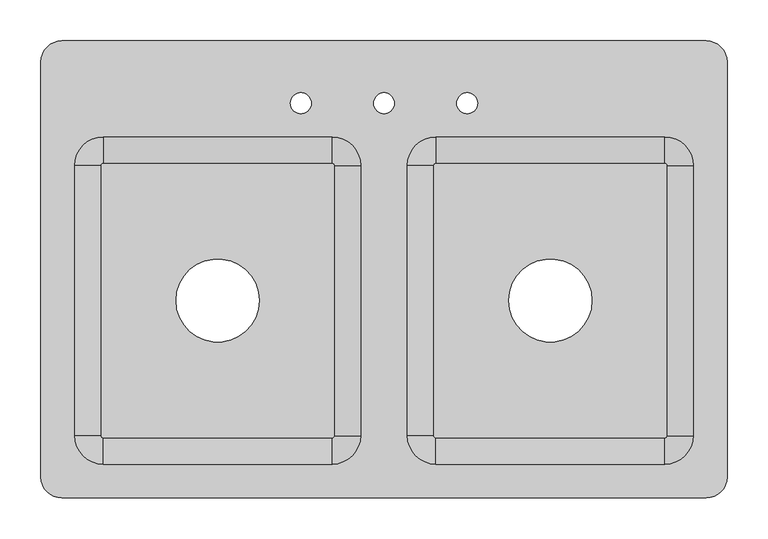
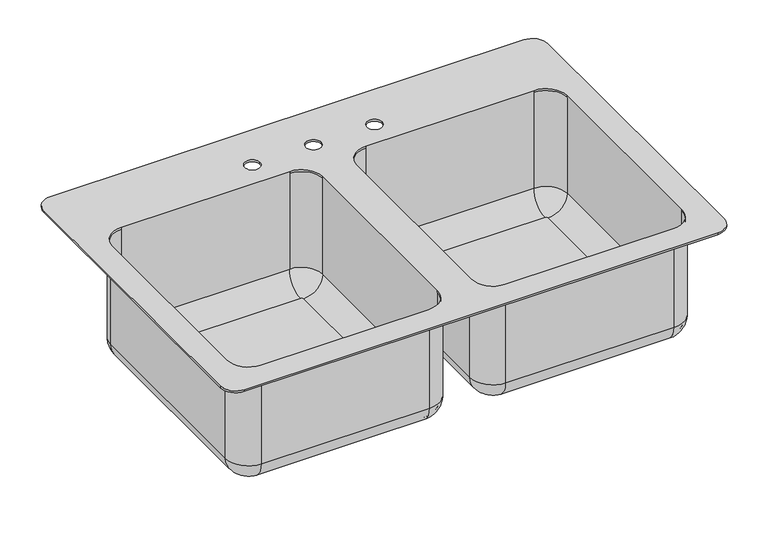
"""IFC4 building model written with IfcOpenShell, lengths in millimetres: proxy geometry, Double_Bowl_Kitchen_Sink_w_Delta_Faucet_and_drains_14175 : Double_Bowl_Kitchen_Sink_w_Delta_Faucet_and_drains_14175."""

import ifcopenshell
import ifcopenshell.guid

model = None  # the IFC model being written
_history = None  # IfcOwnerHistory: only IFC2X3 demands one
_inside = {}  # id of a spatial element -> (the spatial element, [elements in it])
_under = {}  # id of a project, library or spatial element -> (it, [spatial elements below it])
_declared = {}  # id of a project -> (the project, [libraries it declares])
_typed = {}  # id of a type object -> (the type object, [elements of that type])
_made_of = {}  # id of a material, layer set ... -> (it, [elements and type objects made of it])


def new_model(schema):
    """Start an empty IFC model of exactly this schema.

    Asked for "IFC4X3", IfcOpenShell would pick the latest addendum, in which some entities
    have other attributes; the version numbers below select the first issue.
    IFC2X3 requires an IfcOwnerHistory on every rooted entity: one is made here for all.
    """
    global model, _history
    if schema == "IFC4X3":
        model = ifcopenshell.file(schema_version=(4, 3, 0, 0))
    else:
        model = ifcopenshell.file(schema=schema)
    _inside.clear()
    _under.clear()
    _declared.clear()
    _typed.clear()
    _made_of.clear()
    _history = None
    if model.schema == "IFC2X3":
        org = make("IfcOrganization", Name="unknown")
        user = make(
            "IfcPersonAndOrganization",
            ThePerson=make("IfcPerson", FamilyName="unknown"),
            TheOrganization=org,
        )
        app = make(
            "IfcApplication",
            ApplicationDeveloper=org,
            Version="unknown",
            ApplicationFullName="unknown",
            ApplicationIdentifier="unknown",
        )
        _history = make(
            "IfcOwnerHistory",
            OwningUser=user,
            OwningApplication=app,
            ChangeAction="ADDED",
            CreationDate=0,
        )
    return model


def make(cls, **values):
    """One entity of the class cls with the attributes given. An attribute that is None is left unset."""
    return model.create_entity(
        cls, **{name: value for name, value in values.items() if value is not None}
    )


def rooted(cls, **values):
    """An entity with a GlobalId (a new one), such as an element, a storey or a relation."""
    return make(cls, GlobalId=ifcopenshell.guid.new(), OwnerHistory=_history, **values)


def si_unit(unit_type, name, prefix=None):
    """IfcSIUnit, for example si_unit("LENGTHUNIT", "METRE", prefix="MILLI")."""
    return make("IfcSIUnit", UnitType=unit_type, Prefix=prefix, Name=name)


def assignment(units):
    """IfcUnitAssignment: the units of a project."""
    return None if units is None else make("IfcUnitAssignment", Units=units)


def point(xyz):
    """IfcCartesianPoint."""
    return None if xyz is None else make("IfcCartesianPoint", Coordinates=xyz)


def direction(xyz):
    """IfcDirection."""
    return None if xyz is None else make("IfcDirection", DirectionRatios=xyz)


def frame(location, z_axis=None, x_axis=None):
    """IfcAxis2Placement3D, a coordinate frame: its origin and axes. An axis left out is left unset."""
    return make(
        "IfcAxis2Placement3D",
        Location=point(location),
        Axis=direction(z_axis),
        RefDirection=direction(x_axis),
    )


def origin():
    """The frame at (0, 0, 0) with its axes left unset."""
    return frame((0.0, 0.0, 0.0))


def place(relative_to, where):
    """IfcLocalPlacement: puts the frame where relative to a parent placement (None: the world)."""
    return make(
        "IfcLocalPlacement", PlacementRelTo=relative_to, RelativePlacement=where
    )


def context(
    kind, dimensions, precision=None, world=None, true_north=None, identifier=None
):
    """IfcGeometricRepresentationContext, for example the 3D "Model" context."""
    return make(
        "IfcGeometricRepresentationContext",
        ContextIdentifier=identifier,
        ContextType=kind,
        CoordinateSpaceDimension=dimensions,
        Precision=precision,
        WorldCoordinateSystem=world,
        TrueNorth=true_north,
    )


def project(units=None, contexts=None):
    """IfcProject with its units and contexts."""
    return rooted(
        "IfcProject",
        Name="project",
        RepresentationContexts=contexts,
        UnitsInContext=assignment(units),
    )


def spatial(cls, under=None, at=None, **own):
    """A site, building, storey or space (cls), placed at a placement, below another one or the project."""
    s = rooted(cls, ObjectPlacement=at, **own)
    if under is not None:
        _under.setdefault(under.id(), (under, []))[1].append(s)
    return s


def polyline(points):
    """IfcPolyline through the points."""
    return make("IfcPolyline", Points=[point(p) for p in points])


def circle_curve(where, radius):
    """IfcCircle in the frame where."""
    return make("IfcCircle", Position=where, Radius=radius)


def ellipse_curve(where, semi_axis1, semi_axis2):
    """IfcEllipse in the frame where."""
    return make(
        "IfcEllipse", Position=where, SemiAxis1=semi_axis1, SemiAxis2=semi_axis2
    )


def trimmed(basis, trim1, trim2, sense, master):
    """IfcTrimmedCurve: the piece of a basis curve between two trims."""
    return make(
        "IfcTrimmedCurve",
        BasisCurve=basis,
        Trim1=trim1,
        Trim2=trim2,
        SenseAgreement=sense,
        MasterRepresentation=master,
    )


def shape(context_of_items, identifier, shape_type, items):
    """IfcShapeRepresentation: the items that make up one representation, for example the "Body"."""
    return make(
        "IfcShapeRepresentation",
        ContextOfItems=context_of_items,
        RepresentationIdentifier=identifier,
        RepresentationType=shape_type,
        Items=items,
    )


def source(mapping_origin, context_of_items, identifier, shape_type, items):
    """IfcRepresentationMap: a shape defined once, which mapped items show again and again."""
    return make(
        "IfcRepresentationMap",
        MappingOrigin=mapping_origin,
        MappedRepresentation=shape(context_of_items, identifier, shape_type, items),
    )


def transform(
    local_origin,
    x_axis=None,
    y_axis=None,
    z_axis=None,
    scale=None,
    scale2=None,
    scale3=None,
    uniform=True,
):
    """IfcCartesianTransformationOperator3D, or its non-uniform kind. x_axis, y_axis, z_axis: its Axis1, 2, 3."""
    if uniform:
        return make(
            "IfcCartesianTransformationOperator3D",
            Axis1=direction(x_axis),
            Axis2=direction(y_axis),
            LocalOrigin=point(local_origin),
            Scale=scale,
            Axis3=direction(z_axis),
        )
    return make(
        "IfcCartesianTransformationOperator3DnonUniform",
        Axis1=direction(x_axis),
        Axis2=direction(y_axis),
        LocalOrigin=point(local_origin),
        Scale=scale,
        Axis3=direction(z_axis),
        Scale2=scale2,
        Scale3=scale3,
    )


def mapped(mapping_source, mapping_target):
    """IfcMappedItem: shows the shape of a source again, moved by a transform."""
    return make(
        "IfcMappedItem", MappingSource=mapping_source, MappingTarget=mapping_target
    )


def made_of(thing, what):
    """Note that an element or type object is made of a material, layer set ...; save() writes the relation."""
    if what is not None:
        _made_of.setdefault(what.id(), (what, []))[1].append(thing)
    return thing


def element(
    cls,
    number,
    at=None,
    inside=None,
    cuts=None,
    type_object=None,
    material=None,
    context=None,
    identifier="Body",
    shape_type=None,
    held_by="IfcProductDefinitionShape",
    body=None,
    shapes=None,
    **own,
):
    """One element of the class cls, such as IfcWall. Its Tag is "e" and its number.

    at: its placement. inside: the storey or other place that contains it. cuts: it is an
    opening in that element (IfcRelVoidsElement). A single representation is given by context,
    identifier, shape_type and body (its items); several are given by shapes. held_by: the class
    of the entity that holds the representations. save() writes the other relations.
    """
    e = rooted(cls, Tag="e%d" % number, ObjectPlacement=at, **own)
    if body is not None:
        shapes = [shape(context, identifier, shape_type, body)]
    if shapes is not None:
        e.Representation = make(held_by, Representations=shapes)
    if inside is not None:
        _inside.setdefault(inside.id(), (inside, []))[1].append(e)
    if cuts is not None:
        rooted(
            "IfcRelVoidsElement", RelatingBuildingElement=cuts, RelatedOpeningElement=e
        )
    if type_object is not None:
        _typed.setdefault(type_object.id(), (type_object, []))[1].append(e)
    return made_of(e, material)


def aggregate(whole, parts):
    """IfcRelAggregates: a whole, such as a stair, and the parts it consists of."""
    return rooted("IfcRelAggregates", RelatingObject=whole, RelatedObjects=parts)


def save(model, path):
    """Write the relations noted so far, then the file.

    IfcRelAggregates (storeys below a building ...), IfcRelContainedInSpatialStructure (elements
    in a storey), IfcRelDefinesByType, IfcRelAssociatesMaterial and IfcRelDeclares: one each for
    every whole, place, type object, material and project.
    """
    for whole, parts in _under.values():
        aggregate(whole, parts)
    for where, things in _inside.values():
        rooted(
            "IfcRelContainedInSpatialStructure",
            RelatedElements=things,
            RelatingStructure=where,
        )
    for kind, things in _typed.values():
        rooted("IfcRelDefinesByType", RelatedObjects=things, RelatingType=kind)
    for what, things in _made_of.values():
        rooted("IfcRelAssociatesMaterial", RelatedObjects=things, RelatingMaterial=what)
    for by, libraries in _declared.values():
        rooted("IfcRelDeclares", RelatingContext=by, RelatedDefinitions=libraries)
    model.write(path)


def plane_surface(at):
    """IfcPlane: the flat surface through the origin of the frame at, square to its z axis."""
    return make("IfcPlane", Position=at)


def cylinder_surface(at, radius):
    """IfcCylindricalSurface: all points at the distance radius from the z axis of the frame at."""
    return make("IfcCylindricalSurface", Position=at, Radius=radius)


def revolved_surface(curve, axis_point, axis_direction):
    """IfcSurfaceOfRevolution: the curve turned about the line through axis_point along axis_direction."""
    return make(
        "IfcSurfaceOfRevolution",
        SweptCurve=make("IfcArbitraryOpenProfileDef", ProfileType="CURVE", Curve=curve),
        AxisPosition=make("IfcAxis1Placement", Location=point(axis_point), Axis=direction(axis_direction)),
    )


def advanced_brep(points, edges, surfaces, faces):
    """IfcAdvancedBrep: a solid bounded by faces that lie on surfaces and meet in shared edges.

    An edge is (start, end): straight between two places in points (the first is 0);
    or (start, end, curve); or (start, end, curve, False) where it runs against its curve.
    A face is (place in surfaces, loops), or (place, loops, False) where it looks against
    its surface's normal. A loop lists edges by number (the first is 1), with a minus sign
    where the edge is run from its end to its start. The first loop is the outer one.
    """
    corners = [point(p) for p in points]
    vertices = [make("IfcVertexPoint", VertexGeometry=c) for c in corners]
    made = []
    for start, end, *more in edges:
        made.append(
            make(
                "IfcEdgeCurve",
                EdgeStart=vertices[start],
                EdgeEnd=vertices[end],
                EdgeGeometry=more[0] if more else make("IfcPolyline", Points=[corners[start], corners[end]]),
                SameSense=more[1] if len(more) > 1 else True,
            )
        )
    hull = []
    for where, loops, *sense in faces:
        bounds = []
        for j, loop in enumerate(loops):
            ring = [make("IfcOrientedEdge", EdgeElement=made[abs(k) - 1], Orientation=k > 0) for k in loop]
            bounds.append(
                make(
                    "IfcFaceOuterBound" if j == 0 else "IfcFaceBound",
                    Bound=make("IfcEdgeLoop", EdgeList=ring),
                    Orientation=True,
                )
            )
        hull.append(make("IfcAdvancedFace", Bounds=bounds, FaceSurface=surfaces[where], SameSense=sense[0] if sense else True))
    return make("IfcAdvancedBrep", Outer=make("IfcClosedShell", CfsFaces=hull))


def specialty_equipment_74882aa0(model_context):
    return source(origin(), model_context, "Body", "AdvancedBrep", [
        advanced_brep(
        [(342.9, 161.925, 0.0), (342.9, 161.925, -168.275), (377.825, 127.0, -168.275), (377.825, 127.0, 0.0), (381.0, 127.0, -168.275), (342.9, 165.1, -168.275), (342.9, 165.1, 0.0), (381.0, 127.0, 0.0), (346.075, 127.0, -203.2), (342.9, 130.175, -203.2), (342.9, 130.175, -200.025), (346.075, 127.0, -200.025), (381.0, -203.2, 0.0), (381.0, -203.2, -168.275), (346.075, -203.2, -203.2), (346.075, -203.2, -200.025), (377.825, -203.2, -168.275), (377.825, -203.2, 0.0), (342.9, -238.125, -168.275), (342.9, -238.125, 0.0), (342.9, -241.3, 0.0), (342.9, -241.3, -168.275), (342.9, -206.375, -203.2), (342.9, -206.375, -200.025), (63.5, -241.3, 0.0), (63.5, -241.3, -168.275), (63.5, -206.375, -203.2), (63.5, -206.375, -200.025), (63.5, -238.125, -168.275), (63.5, -238.125, 0.0), (28.575, -203.2, -168.275), (28.575, -203.2, 0.0), (25.4, -203.2, 0.0), (25.4, -203.2, -168.275), (60.325, -203.2, -203.2), (60.325, -203.2, -200.025), (25.4, 127.0, 0.0), (25.4, 127.0, -168.275), (60.325, 127.0, -203.2), (60.325, 127.0, -200.025), (28.575, 127.0, -168.275), (28.575, 127.0, 0.0), (63.5, 161.925, -168.275), (63.5, 161.925, 0.0), (63.5, 165.1, 0.0), (63.5, 165.1, -168.275), (63.5, 130.175, -203.2), (63.5, 130.175, -200.025), (393.7, 279.4, 3.175), (-393.7, 279.4, 3.175), (-419.1, 254.0, 3.175), (-419.1, -254.0, 3.175), (-393.7, -279.4, 3.175), (393.7, -279.4, 3.175), (419.1, -254.0, 3.175), (419.1, 254.0, 3.175), (-88.9, 203.2, 3.175), (-114.3, 203.2, 3.175), (12.7, 203.2, 3.175), (-12.7, 203.2, 3.175), (114.3, 203.2, 3.175), (88.9, 203.2, 3.175), (-342.9, 161.925, 3.175), (-63.5, 161.925, 3.175), (-28.575, 127.0, 3.175), (-28.575, -203.2, 3.175), (-63.5, -238.125, 3.175), (-342.9, -238.125, 3.175), (-377.825, -203.2, 3.175), (-377.825, 127.0, 3.175), (28.575, 127.0, 3.175), (63.5, 161.925, 3.175), (342.9, 161.925, 3.175), (377.825, 127.0, 3.175), (377.825, -203.2, 3.175), (342.9, -238.125, 3.175), (63.5, -238.125, 3.175), (28.575, -203.2, 3.175), (393.7, 279.4, 0.0), (419.1, 254.0, 0.0), (419.1, -254.0, 0.0), (393.7, -279.4, 0.0), (-393.7, -279.4, 0.0), (-419.1, -254.0, 0.0), (-419.1, 254.0, 0.0), (-393.7, 279.4, 0.0), (-114.3, 203.2, 0.0), (-88.9, 203.2, 0.0), (-12.7, 203.2, 0.0), (12.7, 203.2, 0.0), (88.9, 203.2, 0.0), (114.3, 203.2, 0.0), (-25.4, 127.0, 0.0), (-63.5, 165.1, 0.0), (-342.9, 165.1, 0.0), (-381.0, 127.0, 0.0), (-381.0, -203.2, 0.0), (-342.9, -241.3, 0.0), (-63.5, -241.3, 0.0), (-25.4, -203.2, 0.0), (-63.5, 161.925, 0.0), (-342.9, 161.925, 0.0), (-342.9, 161.925, -168.275), (-63.5, 161.925, -168.275), (-377.825, 127.0, 0.0), (-377.825, -203.2, 0.0), (-377.825, -203.2, -168.275), (-377.825, 127.0, -168.275), (-342.9, -238.125, 0.0), (-63.5, -238.125, 0.0), (-63.5, -238.125, -168.275), (-342.9, -238.125, -168.275), (-28.575, -203.2, 0.0), (-28.575, 127.0, 0.0), (-28.575, 127.0, -168.275), (-28.575, -203.2, -168.275), (-25.4, 127.0, -168.275), (-63.5, 165.1, -168.275), (-60.325, 127.0, -203.2), (-63.5, 130.175, -203.2), (-63.5, 130.175, -200.025), (-60.325, 127.0, -200.025), (-25.4, -203.2, -168.275), (-60.325, -203.2, -203.2), (-60.325, -203.2, -200.025), (-63.5, -241.3, -168.275), (-63.5, -206.375, -203.2), (-63.5, -206.375, -200.025), (-342.9, -241.3, -168.275), (-342.9, -206.375, -203.2), (-342.9, -206.375, -200.025), (-381.0, -203.2, -168.275), (-346.075, -203.2, -203.2), (-346.075, -203.2, -200.025), (-381.0, 127.0, -168.275), (-346.075, 127.0, -203.2), (-346.075, 127.0, -200.025), (-342.9, 165.1, -168.275), (-342.9, 130.175, -203.2), (-342.9, 130.175, -200.025), (152.4, -38.1, -200.025), (254.0, -38.1, -200.025), (-254.0, -38.1, -200.025), (-152.4, -38.1, -200.025), (254.0, -38.1, -203.2), (152.4, -38.1, -203.2), (-152.4, -38.1, -203.2), (-254.0, -38.1, -203.2)],
        [
            (0, 1),
            (1, 2, circle_curve(frame((342.9, 127.0, -168.275), z_axis=(0.0, 0.0, -1.0), x_axis=(0.0, 1.0, 0.0)), 34.925)),
            (2, 3),
            (3, 0, circle_curve(frame((342.9, 127.0, 0.0), z_axis=(0.0, 0.0, 1.0), x_axis=(0.0, 1.0, 0.0)), 34.925)),
            (4, 5, circle_curve(frame((342.9, 127.0, -168.275), z_axis=(0.0, 0.0, 1.0), x_axis=(0.0, 1.0, 0.0)), 38.1)),
            (5, 6),
            (6, 7, circle_curve(frame((342.9, 127.0, 0.0), z_axis=(0.0, 0.0, -1.0), x_axis=(0.0, 1.0, 0.0)), 38.1)),
            (7, 4),
            (4, 8, circle_curve(frame((346.075, 127.0, -168.275), z_axis=(0.0, 1.0, 0.0), x_axis=(1.0, 0.0, 0.0)), 34.925)),
            (8, 9, circle_curve(frame((342.9, 127.0, -203.2), z_axis=(0.0, 0.0, 1.0), x_axis=(0.0, 1.0, 0.0)), 3.175)),
            (9, 5, circle_curve(frame((342.9, 130.175, -168.275), z_axis=(1.0, 0.0, 0.0), x_axis=(0.0, 1.0, 0.0)), 34.925)),
            (1, 10, circle_curve(frame((342.9, 130.175, -168.275), z_axis=(-1.0, 0.0, 0.0), x_axis=(0.0, 1.0, 0.0)), 31.75)),
            (10, 11, circle_curve(frame((342.9, 127.0, -200.025), z_axis=(0.0, 0.0, -1.0), x_axis=(0.0, 1.0, 0.0)), 3.175)),
            (11, 2, circle_curve(frame((346.075, 127.0, -168.275), z_axis=(0.0, -1.0, 0.0), x_axis=(1.0, 0.0, 0.0)), 31.75)),
            (7, 12),
            (12, 13),
            (13, 4),
            (13, 14, circle_curve(frame((346.075, -203.2, -168.275), z_axis=(0.0, 1.0, 0.0), x_axis=(1.0, 0.0, 0.0)), 34.925)),
            (14, 8),
            (11, 15),
            (15, 16, circle_curve(frame((346.075, -203.2, -168.275), z_axis=(0.0, -1.0, 0.0), x_axis=(1.0, 0.0, 0.0)), 31.75)),
            (16, 2),
            (17, 16),
            (16, 18, circle_curve(frame((342.9, -203.2, -168.275), z_axis=(0.0, 0.0, -1.0), x_axis=(1.0, 0.0, 0.0)), 34.925)),
            (18, 19),
            (19, 17, circle_curve(frame((342.9, -203.2, 0.0), z_axis=(0.0, 0.0, 1.0), x_axis=(1.0, 0.0, 0.0)), 34.925)),
            (12, 20, circle_curve(frame((342.9, -203.2, 0.0), z_axis=(0.0, 0.0, -1.0), x_axis=(1.0, 0.0, 0.0)), 38.1)),
            (20, 21),
            (21, 13, circle_curve(frame((342.9, -203.2, -168.275), z_axis=(0.0, 0.0, 1.0), x_axis=(1.0, 0.0, 0.0)), 38.1)),
            (21, 22, circle_curve(frame((342.9, -206.375, -168.275), z_axis=(1.0, 0.0, 0.0), x_axis=(0.0, -1.0, 0.0)), 34.925)),
            (22, 14, circle_curve(frame((342.9, -203.2, -203.2), z_axis=(0.0, 0.0, 1.0), x_axis=(1.0, 0.0, 0.0)), 3.175)),
            (15, 23, circle_curve(frame((342.9, -203.2, -200.025), z_axis=(0.0, 0.0, -1.0), x_axis=(1.0, 0.0, 0.0)), 3.175)),
            (23, 18, circle_curve(frame((342.9, -206.375, -168.275), z_axis=(-1.0, 0.0, 0.0), x_axis=(0.0, -1.0, 0.0)), 31.75)),
            (20, 24),
            (24, 25),
            (25, 21),
            (25, 26, circle_curve(frame((63.5, -206.375, -168.275), z_axis=(1.0, 0.0, 0.0), x_axis=(0.0, -1.0, 0.0)), 34.925)),
            (26, 22),
            (23, 27),
            (27, 28, circle_curve(frame((63.5, -206.375, -168.275), z_axis=(-1.0, 0.0, 0.0), x_axis=(0.0, -1.0, 0.0)), 31.75)),
            (28, 18),
            (29, 28),
            (28, 30, circle_curve(frame((63.5, -203.2, -168.275), z_axis=(0.0, 0.0, -1.0), x_axis=(0.0, -1.0, 0.0)), 34.925)),
            (30, 31),
            (31, 29, circle_curve(frame((63.5, -203.2, 0.0), z_axis=(0.0, 0.0, 1.0), x_axis=(0.0, -1.0, 0.0)), 34.925)),
            (24, 32, circle_curve(frame((63.5, -203.2, 0.0), z_axis=(0.0, 0.0, -1.0), x_axis=(0.0, -1.0, 0.0)), 38.1)),
            (32, 33),
            (33, 25, circle_curve(frame((63.5, -203.2, -168.275), z_axis=(0.0, 0.0, 1.0), x_axis=(0.0, -1.0, 0.0)), 38.1)),
            (33, 34, circle_curve(frame((60.325, -203.2, -168.275), z_axis=(0.0, -1.0, 0.0), x_axis=(-1.0, 0.0, 0.0)), 34.925)),
            (34, 26, circle_curve(frame((63.5, -203.2, -203.2), z_axis=(0.0, 0.0, 1.0), x_axis=(0.0, -1.0, 0.0)), 3.175)),
            (27, 35, circle_curve(frame((63.5, -203.2, -200.025), z_axis=(0.0, 0.0, -1.0), x_axis=(0.0, -1.0, 0.0)), 3.175)),
            (35, 30, circle_curve(frame((60.325, -203.2, -168.275), z_axis=(0.0, 1.0, 0.0), x_axis=(-1.0, 0.0, 0.0)), 31.75)),
            (32, 36),
            (36, 37),
            (37, 33),
            (37, 38, circle_curve(frame((60.325, 127.0, -168.275), z_axis=(0.0, -1.0, 0.0), x_axis=(-1.0, 0.0, 0.0)), 34.925)),
            (38, 34),
            (35, 39),
            (39, 40, circle_curve(frame((60.325, 127.0, -168.275), z_axis=(0.0, 1.0, 0.0), x_axis=(-1.0, 0.0, 0.0)), 31.75)),
            (40, 30),
            (41, 40),
            (40, 42, circle_curve(frame((63.5, 127.0, -168.275), z_axis=(0.0, 0.0, -1.0), x_axis=(-1.0, 0.0, 0.0)), 34.925)),
            (42, 43),
            (43, 41, circle_curve(frame((63.5, 127.0, 0.0), z_axis=(0.0, 0.0, 1.0), x_axis=(-1.0, 0.0, 0.0)), 34.925)),
            (36, 44, circle_curve(frame((63.5, 127.0, 0.0), z_axis=(0.0, 0.0, -1.0), x_axis=(-1.0, 0.0, 0.0)), 38.1)),
            (44, 45),
            (45, 37, circle_curve(frame((63.5, 127.0, -168.275), z_axis=(0.0, 0.0, 1.0), x_axis=(-1.0, 0.0, 0.0)), 38.1)),
            (45, 46, circle_curve(frame((63.5, 130.175, -168.275), z_axis=(-1.0, 0.0, 0.0), x_axis=(0.0, 1.0, 0.0)), 34.925)),
            (46, 38, circle_curve(frame((63.5, 127.0, -203.2), z_axis=(0.0, 0.0, 1.0), x_axis=(-1.0, 0.0, 0.0)), 3.175)),
            (39, 47, circle_curve(frame((63.5, 127.0, -200.025), z_axis=(0.0, 0.0, -1.0), x_axis=(-1.0, 0.0, 0.0)), 3.175)),
            (47, 42, circle_curve(frame((63.5, 130.175, -168.275), z_axis=(1.0, 0.0, 0.0), x_axis=(0.0, 1.0, 0.0)), 31.75)),
            (5, 45),
            (44, 6),
            (9, 46),
            (1, 42),
            (47, 10),
            (48, 49),
            (49, 50, circle_curve(frame((-393.7, 254.0, 3.175), z_axis=(0.0, 0.0, 1.0), x_axis=(1.0, 0.0, 0.0)), 25.4)),
            (50, 51),
            (51, 52, circle_curve(frame((-393.7, -254.0, 3.175), z_axis=(0.0, 0.0, 1.0), x_axis=(1.0, 0.0, 0.0)), 25.4)),
            (52, 53),
            (53, 54, circle_curve(frame((393.7, -254.0, 3.175), z_axis=(0.0, 0.0, 1.0), x_axis=(1.0, 0.0, 0.0)), 25.4)),
            (54, 55),
            (55, 48, circle_curve(frame((393.7, 254.0, 3.175), z_axis=(0.0, 0.0, 1.0), x_axis=(1.0, 0.0, 0.0)), 25.4)),
            (56, 57, circle_curve(frame((-101.6, 203.2, 3.175), z_axis=(0.0, 0.0, -1.0), x_axis=(1.0, 0.0, 0.0)), 12.7)),
            (57, 56, circle_curve(frame((-101.6, 203.2, 3.175), z_axis=(0.0, 0.0, -1.0), x_axis=(1.0, 0.0, 0.0)), 12.7)),
            (58, 59, circle_curve(frame((0.0, 203.2, 3.175), z_axis=(0.0, 0.0, -1.0), x_axis=(1.0, 0.0, 0.0)), 12.7)),
            (59, 58, circle_curve(frame((0.0, 203.2, 3.175), z_axis=(0.0, 0.0, -1.0), x_axis=(1.0, 0.0, 0.0)), 12.7)),
            (60, 61, circle_curve(frame((101.6, 203.2, 3.175), z_axis=(0.0, 0.0, -1.0), x_axis=(1.0, 0.0, 0.0)), 12.7)),
            (61, 60, circle_curve(frame((101.6, 203.2, 3.175), z_axis=(0.0, 0.0, -1.0), x_axis=(1.0, 0.0, 0.0)), 12.7)),
            (62, 63),
            (63, 64, circle_curve(frame((-63.5, 127.0, 3.175), z_axis=(0.0, 0.0, -1.0), x_axis=(1.0, 0.0, 0.0)), 34.925)),
            (64, 65),
            (65, 66, circle_curve(frame((-63.5, -203.2, 3.175), z_axis=(0.0, 0.0, -1.0), x_axis=(1.0, 0.0, 0.0)), 34.925)),
            (66, 67),
            (67, 68, circle_curve(frame((-342.9, -203.2, 3.175), z_axis=(0.0, 0.0, -1.0), x_axis=(1.0, 0.0, 0.0)), 34.925)),
            (68, 69),
            (69, 62, circle_curve(frame((-342.9, 127.0, 3.175), z_axis=(0.0, 0.0, -1.0), x_axis=(1.0, 0.0, 0.0)), 34.925)),
            (70, 71, circle_curve(frame((63.5, 127.0, 3.175), z_axis=(0.0, 0.0, -1.0), x_axis=(1.0, 0.0, 0.0)), 34.925)),
            (71, 72),
            (72, 73, circle_curve(frame((342.9, 127.0, 3.175), z_axis=(0.0, 0.0, -1.0), x_axis=(1.0, 0.0, 0.0)), 34.925)),
            (73, 74),
            (74, 75, circle_curve(frame((342.9, -203.2, 3.175), z_axis=(0.0, 0.0, -1.0), x_axis=(1.0, 0.0, 0.0)), 34.925)),
            (75, 76),
            (76, 77, circle_curve(frame((63.5, -203.2, 3.175), z_axis=(0.0, 0.0, -1.0), x_axis=(1.0, 0.0, 0.0)), 34.925)),
            (77, 70),
            (78, 79, circle_curve(frame((393.7, 254.0, 0.0), z_axis=(0.0, 0.0, -1.0), x_axis=(1.0, 0.0, 0.0)), 25.4)),
            (79, 80),
            (80, 81, circle_curve(frame((393.7, -254.0, 0.0), z_axis=(0.0, 0.0, -1.0), x_axis=(1.0, 0.0, 0.0)), 25.4)),
            (81, 82),
            (82, 83, circle_curve(frame((-393.7, -254.0, 0.0), z_axis=(0.0, 0.0, -1.0), x_axis=(1.0, 0.0, 0.0)), 25.4)),
            (83, 84),
            (84, 85, circle_curve(frame((-393.7, 254.0, 0.0), z_axis=(0.0, 0.0, -1.0), x_axis=(1.0, 0.0, 0.0)), 25.4)),
            (85, 78),
            (86, 87, circle_curve(frame((-101.6, 203.2, 0.0), z_axis=(0.0, 0.0, 1.0), x_axis=(1.0, 0.0, 0.0)), 12.7)),
            (87, 86, circle_curve(frame((-101.6, 203.2, 0.0), z_axis=(0.0, 0.0, 1.0), x_axis=(1.0, 0.0, 0.0)), 12.7)),
            (88, 89, circle_curve(frame((0.0, 203.2, 0.0), z_axis=(0.0, 0.0, 1.0), x_axis=(1.0, 0.0, 0.0)), 12.7)),
            (89, 88, circle_curve(frame((0.0, 203.2, 0.0), z_axis=(0.0, 0.0, 1.0), x_axis=(1.0, 0.0, 0.0)), 12.7)),
            (90, 91, circle_curve(frame((101.6, 203.2, 0.0), z_axis=(0.0, 0.0, 1.0), x_axis=(1.0, 0.0, 0.0)), 12.7)),
            (91, 90, circle_curve(frame((101.6, 203.2, 0.0), z_axis=(0.0, 0.0, 1.0), x_axis=(1.0, 0.0, 0.0)), 12.7)),
            (92, 93, circle_curve(frame((-63.5, 127.0, 0.0), z_axis=(0.0, 0.0, 1.0), x_axis=(0.0, 1.0, 0.0)), 38.1)),
            (93, 94),
            (94, 95, circle_curve(frame((-342.9, 127.0, 0.0), z_axis=(0.0, 0.0, 1.0), x_axis=(-1.0, 0.0, 0.0)), 38.1)),
            (95, 96),
            (96, 97, circle_curve(frame((-342.9, -203.2, 0.0), z_axis=(0.0, 0.0, 1.0), x_axis=(0.0, -1.0, 0.0)), 38.1)),
            (97, 98),
            (98, 99, circle_curve(frame((-63.5, -203.2, 0.0), z_axis=(0.0, 0.0, 1.0), x_axis=(1.0, 0.0, 0.0)), 38.1)),
            (99, 92),
            (48, 78),
            (85, 49),
            (84, 50),
            (83, 51),
            (82, 52),
            (81, 53),
            (80, 54),
            (79, 55),
            (86, 57),
            (56, 87),
            (88, 59),
            (58, 89),
            (90, 61),
            (60, 91),
            (100, 63),
            (62, 101),
            (101, 102),
            (102, 103),
            (103, 100),
            (69, 104),
            (104, 101, circle_curve(frame((-342.9, 127.0, 0.0), z_axis=(0.0, 0.0, -1.0), x_axis=(1.0, 0.0, 0.0)), 34.925)),
            (68, 105),
            (105, 106),
            (106, 107),
            (107, 104),
            (67, 108),
            (108, 105, circle_curve(frame((-342.9, -203.2, 0.0), z_axis=(0.0, 0.0, -1.0), x_axis=(1.0, 0.0, 0.0)), 34.925)),
            (66, 109),
            (109, 110),
            (110, 111),
            (111, 108),
            (65, 112),
            (112, 109, circle_curve(frame((-63.5, -203.2, 0.0), z_axis=(0.0, 0.0, -1.0), x_axis=(1.0, 0.0, 0.0)), 34.925)),
            (64, 113),
            (113, 114),
            (114, 115),
            (115, 112),
            (100, 113, circle_curve(frame((-63.5, 127.0, 0.0), z_axis=(0.0, 0.0, -1.0), x_axis=(1.0, 0.0, 0.0)), 34.925)),
            (43, 71),
            (70, 41),
            (77, 31),
            (76, 29),
            (75, 19),
            (74, 17),
            (73, 3),
            (72, 0),
            (103, 114, circle_curve(frame((-63.5, 127.0, -168.275), z_axis=(0.0, 0.0, -1.0), x_axis=(0.0, 1.0, 0.0)), 34.925)),
            (116, 117, circle_curve(frame((-63.5, 127.0, -168.275), z_axis=(0.0, 0.0, 1.0), x_axis=(0.0, 1.0, 0.0)), 38.1)),
            (117, 93),
            (92, 116),
            (116, 118, circle_curve(frame((-60.325, 127.0, -168.275), z_axis=(0.0, 1.0, 0.0), x_axis=(1.0, 0.0, 0.0)), 34.925)),
            (118, 119, circle_curve(frame((-63.5, 127.0, -203.2), z_axis=(0.0, 0.0, 1.0), x_axis=(0.0, 1.0, 0.0)), 3.175)),
            (119, 117, circle_curve(frame((-63.5, 130.175, -168.275), z_axis=(1.0, 0.0, 0.0), x_axis=(0.0, 1.0, 0.0)), 34.925)),
            (103, 120, circle_curve(frame((-63.5, 130.175, -168.275), z_axis=(-1.0, 0.0, 0.0), x_axis=(0.0, 1.0, 0.0)), 31.75)),
            (120, 121, circle_curve(frame((-63.5, 127.0, -200.025), z_axis=(0.0, 0.0, -1.0), x_axis=(0.0, 1.0, 0.0)), 3.175)),
            (121, 114, circle_curve(frame((-60.325, 127.0, -168.275), z_axis=(0.0, -1.0, 0.0), x_axis=(1.0, 0.0, 0.0)), 31.75)),
            (99, 122),
            (122, 116),
            (122, 123, circle_curve(frame((-60.325, -203.2, -168.275), z_axis=(0.0, 1.0, 0.0), x_axis=(1.0, 0.0, 0.0)), 34.925)),
            (123, 118),
            (121, 124),
            (124, 115, circle_curve(frame((-60.325, -203.2, -168.275), z_axis=(0.0, -1.0, 0.0), x_axis=(1.0, 0.0, 0.0)), 31.75)),
            (115, 110, circle_curve(frame((-63.5, -203.2, -168.275), z_axis=(0.0, 0.0, -1.0), x_axis=(1.0, 0.0, 0.0)), 34.925)),
            (98, 125),
            (125, 122, circle_curve(frame((-63.5, -203.2, -168.275), z_axis=(0.0, 0.0, 1.0), x_axis=(1.0, 0.0, 0.0)), 38.1)),
            (125, 126, circle_curve(frame((-63.5, -206.375, -168.275), z_axis=(1.0, 0.0, 0.0), x_axis=(0.0, -1.0, 0.0)), 34.925)),
            (126, 123, circle_curve(frame((-63.5, -203.2, -203.2), z_axis=(0.0, 0.0, 1.0), x_axis=(1.0, 0.0, 0.0)), 3.175)),
            (124, 127, circle_curve(frame((-63.5, -203.2, -200.025), z_axis=(0.0, 0.0, -1.0), x_axis=(1.0, 0.0, 0.0)), 3.175)),
            (127, 110, circle_curve(frame((-63.5, -206.375, -168.275), z_axis=(-1.0, 0.0, 0.0), x_axis=(0.0, -1.0, 0.0)), 31.75)),
            (97, 128),
            (128, 125),
            (128, 129, circle_curve(frame((-342.9, -206.375, -168.275), z_axis=(1.0, 0.0, 0.0), x_axis=(0.0, -1.0, 0.0)), 34.925)),
            (129, 126),
            (127, 130),
            (130, 111, circle_curve(frame((-342.9, -206.375, -168.275), z_axis=(-1.0, 0.0, 0.0), x_axis=(0.0, -1.0, 0.0)), 31.75)),
            (111, 106, circle_curve(frame((-342.9, -203.2, -168.275), z_axis=(0.0, 0.0, -1.0), x_axis=(0.0, -1.0, 0.0)), 34.925)),
            (96, 131),
            (131, 128, circle_curve(frame((-342.9, -203.2, -168.275), z_axis=(0.0, 0.0, 1.0), x_axis=(0.0, -1.0, 0.0)), 38.1)),
            (131, 132, circle_curve(frame((-346.075, -203.2, -168.275), z_axis=(0.0, -1.0, 0.0), x_axis=(-1.0, 0.0, 0.0)), 34.925)),
            (132, 129, circle_curve(frame((-342.9, -203.2, -203.2), z_axis=(0.0, 0.0, 1.0), x_axis=(0.0, -1.0, 0.0)), 3.175)),
            (130, 133, circle_curve(frame((-342.9, -203.2, -200.025), z_axis=(0.0, 0.0, -1.0), x_axis=(0.0, -1.0, 0.0)), 3.175)),
            (133, 106, circle_curve(frame((-346.075, -203.2, -168.275), z_axis=(0.0, 1.0, 0.0), x_axis=(-1.0, 0.0, 0.0)), 31.75)),
            (95, 134),
            (134, 131),
            (134, 135, circle_curve(frame((-346.075, 127.0, -168.275), z_axis=(0.0, -1.0, 0.0), x_axis=(-1.0, 0.0, 0.0)), 34.925)),
            (135, 132),
            (133, 136),
            (136, 107, circle_curve(frame((-346.075, 127.0, -168.275), z_axis=(0.0, 1.0, 0.0), x_axis=(-1.0, 0.0, 0.0)), 31.75)),
            (107, 102, circle_curve(frame((-342.9, 127.0, -168.275), z_axis=(0.0, 0.0, -1.0), x_axis=(-1.0, 0.0, 0.0)), 34.925)),
            (94, 137),
            (137, 134, circle_curve(frame((-342.9, 127.0, -168.275), z_axis=(0.0, 0.0, 1.0), x_axis=(-1.0, 0.0, 0.0)), 38.1)),
            (137, 138, circle_curve(frame((-342.9, 130.175, -168.275), z_axis=(-1.0, 0.0, 0.0), x_axis=(0.0, 1.0, 0.0)), 34.925)),
            (138, 135, circle_curve(frame((-342.9, 127.0, -203.2), z_axis=(0.0, 0.0, 1.0), x_axis=(-1.0, 0.0, 0.0)), 3.175)),
            (136, 139, circle_curve(frame((-342.9, 127.0, -200.025), z_axis=(0.0, 0.0, -1.0), x_axis=(-1.0, 0.0, 0.0)), 3.175)),
            (139, 102, circle_curve(frame((-342.9, 130.175, -168.275), z_axis=(1.0, 0.0, 0.0), x_axis=(0.0, 1.0, 0.0)), 31.75)),
            (117, 137),
            (119, 138),
            (139, 120),
            (140, 141, circle_curve(frame((203.2, -38.1, -200.025), z_axis=(0.0, 0.0, -1.0), x_axis=(-1.0, 0.0, 0.0)), 50.8)),
            (141, 140, circle_curve(frame((203.2, -38.1, -200.025), z_axis=(0.0, 0.0, -1.0), x_axis=(-1.0, 0.0, 0.0)), 50.8)),
            (142, 143, circle_curve(frame((-203.2, -38.1, -200.025), z_axis=(0.0, 0.0, -1.0), x_axis=(-1.0, 0.0, 0.0)), 50.8)),
            (143, 142, circle_curve(frame((-203.2, -38.1, -200.025), z_axis=(0.0, 0.0, -1.0), x_axis=(-1.0, 0.0, 0.0)), 50.8)),
            (144, 145, circle_curve(frame((203.2, -38.1, -203.2), z_axis=(0.0, 0.0, 1.0), x_axis=(-1.0, 0.0, 0.0)), 50.8)),
            (145, 144, circle_curve(frame((203.2, -38.1, -203.2), z_axis=(0.0, 0.0, 1.0), x_axis=(-1.0, 0.0, 0.0)), 50.8)),
            (146, 147, circle_curve(frame((-203.2, -38.1, -203.2), z_axis=(0.0, 0.0, 1.0), x_axis=(-1.0, 0.0, 0.0)), 50.8)),
            (147, 146, circle_curve(frame((-203.2, -38.1, -203.2), z_axis=(0.0, 0.0, 1.0), x_axis=(-1.0, 0.0, 0.0)), 50.8)),
            (144, 141),
            (140, 145),
            (146, 143),
            (142, 147),
        ],
        [
            revolved_surface(polyline([(342.9, 161.925, -168.275), (342.9, 161.925, 0.0)]), (342.9, 127.0, 0.0), (0.0, 0.0, -1.0)),
            cylinder_surface(frame((342.9, 127.0, 0.0), z_axis=(0.0, 0.0, -1.0), x_axis=(0.0, 1.0, 0.0)), 38.1),
            revolved_surface(trimmed(ellipse_curve(frame((342.9, 130.175, -168.275), z_axis=(-1.0, 0.0, 0.0), x_axis=(0.0, 1.0, 0.0)), 34.925, 34.925), [point((342.9, 165.1, -168.275))], [point((342.9, 130.175, -203.2))], True, "CARTESIAN"), (342.9, 127.0, 0.0), (0.0, 0.0, -1.0)),
            revolved_surface(trimmed(ellipse_curve(frame((342.9, 130.175, -168.275), z_axis=(1.0, 0.0, 0.0), x_axis=(0.0, 1.0, 0.0)), 31.75, 31.75), [point((342.9, 130.175, -200.025))], [point((342.9, 161.925, -168.275))], True, "CARTESIAN"), (342.9, 127.0, 0.0), (0.0, 0.0, -1.0)),
            plane_surface(frame((381.0, 127.0, 0.0), z_axis=(1.0, 0.0, 0.0), x_axis=(0.0, -1.0, 0.0))),
            cylinder_surface(frame((346.075, 127.0, -168.275), z_axis=(0.0, 1.0, 0.0), x_axis=(1.0, 0.0, 0.0)), 34.925),
            revolved_surface(polyline([(377.825, -203.2, -168.275), (377.825, 127.0, -168.275)]), (346.075, 127.0, -168.275), (0.0, -1.0, 0.0)),
            revolved_surface(polyline([(377.825, -203.2, -168.275), (377.825, -203.2, 0.0)]), (342.9, -203.2, 0.0), (0.0, 0.0, -1.0)),
            cylinder_surface(frame((342.9, -203.2, 0.0), z_axis=(0.0, 0.0, -1.0), x_axis=(1.0, 0.0, 0.0)), 38.1),
            revolved_surface(trimmed(ellipse_curve(frame((346.075, -203.2, -168.275), z_axis=(0.0, 1.0, 0.0), x_axis=(1.0, 0.0, 0.0)), 34.925, 34.925), [point((381.0, -203.2, -168.275))], [point((346.075, -203.2, -203.2))], True, "CARTESIAN"), (342.9, -203.2, 0.0), (0.0, 0.0, -1.0)),
            revolved_surface(trimmed(ellipse_curve(frame((346.075, -203.2, -168.275), z_axis=(0.0, -1.0, 0.0), x_axis=(1.0, 0.0, 0.0)), 31.75, 31.75), [point((346.075, -203.2, -200.025))], [point((377.825, -203.2, -168.275))], True, "CARTESIAN"), (342.9, -203.2, 0.0), (0.0, 0.0, -1.0)),
            plane_surface(frame((342.9, -241.3, 0.0), z_axis=(0.0, -1.0, 0.0), x_axis=(-1.0, 0.0, 0.0))),
            cylinder_surface(frame((342.9, -206.375, -168.275), z_axis=(1.0, 0.0, 0.0), x_axis=(0.0, -1.0, 0.0)), 34.925),
            revolved_surface(polyline([(63.5, -238.125, -168.275), (342.9, -238.125, -168.275)]), (342.9, -206.375, -168.275), (-1.0, 0.0, 0.0)),
            revolved_surface(polyline([(63.5, -238.125, -168.275), (63.5, -238.125, 0.0)]), (63.5, -203.2, 0.0), (0.0, 0.0, -1.0)),
            cylinder_surface(frame((63.5, -203.2, 0.0), z_axis=(0.0, 0.0, -1.0), x_axis=(0.0, -1.0, 0.0)), 38.1),
            revolved_surface(trimmed(ellipse_curve(frame((63.5, -206.375, -168.275), z_axis=(1.0, 0.0, 0.0), x_axis=(0.0, -1.0, 0.0)), 34.925, 34.925), [point((63.5, -241.3, -168.275))], [point((63.5, -206.375, -203.2))], True, "CARTESIAN"), (63.5, -203.2, 0.0), (0.0, 0.0, -1.0)),
            revolved_surface(trimmed(ellipse_curve(frame((63.5, -206.375, -168.275), z_axis=(-1.0, 0.0, 0.0), x_axis=(0.0, -1.0, 0.0)), 31.75, 31.75), [point((63.5, -206.375, -200.025))], [point((63.5, -238.125, -168.275))], True, "CARTESIAN"), (63.5, -203.2, 0.0), (0.0, 0.0, -1.0)),
            plane_surface(frame((25.4, -203.2, 0.0), z_axis=(-1.0, 0.0, 0.0), x_axis=(0.0, 1.0, 0.0))),
            cylinder_surface(frame((60.325, -203.2, -168.275), z_axis=(0.0, -1.0, 0.0), x_axis=(-1.0, 0.0, 0.0)), 34.925),
            revolved_surface(polyline([(28.575000000000003, 127.0, -168.275), (28.575000000000003, -203.2, -168.275)]), (60.325, -203.2, -168.275), (0.0, 1.0, 0.0)),
            revolved_surface(polyline([(28.575000000000003, 127.0, -168.275), (28.575000000000003, 127.0, 0.0)]), (63.5, 127.0, 0.0), (0.0, 0.0, -1.0)),
            cylinder_surface(frame((63.5, 127.0, 0.0), z_axis=(0.0, 0.0, -1.0), x_axis=(-1.0, 0.0, 0.0)), 38.1),
            revolved_surface(trimmed(ellipse_curve(frame((60.325, 127.0, -168.275), z_axis=(0.0, -1.0, 0.0), x_axis=(-1.0, 0.0, 0.0)), 34.925, 34.925), [point((25.4, 127.0, -168.275))], [point((60.325, 127.0, -203.2))], True, "CARTESIAN"), (63.5, 127.0, 0.0), (0.0, 0.0, -1.0)),
            revolved_surface(trimmed(ellipse_curve(frame((60.325, 127.0, -168.275), z_axis=(0.0, 1.0, 0.0), x_axis=(-1.0, 0.0, 0.0)), 31.75, 31.75), [point((60.325, 127.0, -200.025))], [point((28.575, 127.0, -168.275))], True, "CARTESIAN"), (63.5, 127.0, 0.0), (0.0, 0.0, -1.0)),
            plane_surface(frame((63.5, 165.1, 0.0), z_axis=(0.0, 1.0, 0.0), x_axis=(1.0, 0.0, 0.0))),
            cylinder_surface(frame((63.5, 130.175, -168.275), z_axis=(-1.0, 0.0, 0.0), x_axis=(0.0, 1.0, 0.0)), 34.925),
            revolved_surface(polyline([(342.9, 161.925, -168.275), (63.5, 161.925, -168.275)]), (63.5, 130.175, -168.275), (1.0, 0.0, 0.0)),
            plane_surface(frame((-393.7, 279.4, 3.175), z_axis=(0.0, 0.0, 1.0), x_axis=(-1.0, 0.0, 0.0))),
            plane_surface(frame((-393.7, 279.4, 0.0), z_axis=(0.0, 0.0, -1.0), x_axis=(1.0, 0.0, 0.0))),
            plane_surface(frame((393.7, 279.4, 3.175), z_axis=(0.0, 1.0, 0.0), x_axis=(0.0, 0.0, -1.0))),
            cylinder_surface(frame((-393.7, 254.0, 0.0), z_axis=(0.0, 0.0, 1.0), x_axis=(1.0, 0.0, 0.0)), 25.4),
            plane_surface(frame((-419.1, 254.0, 3.175), z_axis=(-1.0, 0.0, 0.0), x_axis=(0.0, 0.0, -1.0))),
            cylinder_surface(frame((-393.7, -254.0, 0.0), z_axis=(0.0, 0.0, 1.0), x_axis=(1.0, 0.0, 0.0)), 25.4),
            plane_surface(frame((-393.7, -279.4, 3.175), z_axis=(0.0, -1.0, 0.0), x_axis=(0.0, 0.0, -1.0))),
            cylinder_surface(frame((393.7, -254.0, 0.0), z_axis=(0.0, 0.0, 1.0), x_axis=(1.0, 0.0, 0.0)), 25.4),
            plane_surface(frame((419.1, -254.0, 3.175), z_axis=(1.0, 0.0, 0.0), x_axis=(0.0, 0.0, -1.0))),
            cylinder_surface(frame((393.7, 254.0, 0.0), z_axis=(0.0, 0.0, 1.0), x_axis=(1.0, 0.0, 0.0)), 25.4),
            revolved_surface(polyline([(-88.89999999999999, 203.2, 3.175), (-88.89999999999999, 203.2, 0.0)]), (-101.6, 203.2, 0.0), (0.0, 0.0, 1.0)),
            revolved_surface(polyline([(12.7, 203.2, 3.175), (12.7, 203.2, 0.0)]), (0.0, 203.2, 0.0), (0.0, 0.0, 1.0)),
            revolved_surface(polyline([(114.3, 203.2, 3.175), (114.3, 203.2, 0.0)]), (101.6, 203.2, 0.0), (0.0, 0.0, 1.0)),
            plane_surface(frame((-63.5, 161.925, 101.6), z_axis=(0.0, -1.0, 0.0), x_axis=(0.0, 0.0, -1.0))),
            revolved_surface(polyline([(-307.97499999999997, 127.0, 3.175), (-307.97499999999997, 127.0, 0.0)]), (-342.9, 127.0, 0.0), (0.0, 0.0, 1.0)),
            plane_surface(frame((-377.825, 127.0, 101.6), z_axis=(1.0, 0.0, 0.0), x_axis=(0.0, 0.0, -1.0))),
            revolved_surface(polyline([(-307.97499999999997, -203.2, 3.175), (-307.97499999999997, -203.2, 0.0)]), (-342.9, -203.2, 0.0), (0.0, 0.0, 1.0)),
            plane_surface(frame((-342.9, -238.125, 101.6), z_axis=(0.0, 1.0, 0.0), x_axis=(0.0, 0.0, -1.0))),
            revolved_surface(polyline([(-28.575000000000003, -203.2, 3.175), (-28.575000000000003, -203.2, 0.0)]), (-63.5, -203.2, 0.0), (0.0, 0.0, 1.0)),
            plane_surface(frame((-28.575, -203.2, 101.6), z_axis=(-1.0, 0.0, 0.0), x_axis=(0.0, 0.0, -1.0))),
            revolved_surface(polyline([(-28.575000000000003, 127.0, 3.175), (-28.575000000000003, 127.0, 0.0)]), (-63.5, 127.0, 0.0), (0.0, 0.0, 1.0)),
            revolved_surface(polyline([(98.425, 127.0, 3.175), (98.425, 127.0, 0.0)]), (63.5, 127.0, 0.0), (0.0, 0.0, 1.0)),
            plane_surface(frame((28.575, 127.0, 101.6), z_axis=(1.0, 0.0, 0.0), x_axis=(0.0, 0.0, -1.0))),
            revolved_surface(polyline([(98.425, -203.2, 3.175), (98.425, -203.2, 0.0)]), (63.5, -203.2, 0.0), (0.0, 0.0, 1.0)),
            plane_surface(frame((63.5, -238.125, 101.6), z_axis=(0.0, 1.0, 0.0), x_axis=(0.0, 0.0, -1.0))),
            revolved_surface(polyline([(377.825, -203.2, 3.175), (377.825, -203.2, 0.0)]), (342.9, -203.2, 0.0), (0.0, 0.0, 1.0)),
            plane_surface(frame((377.825, -203.2, 101.6), z_axis=(-1.0, 0.0, 0.0), x_axis=(0.0, 0.0, -1.0))),
            revolved_surface(polyline([(377.825, 127.0, 3.175), (377.825, 127.0, 0.0)]), (342.9, 127.0, 0.0), (0.0, 0.0, 1.0)),
            plane_surface(frame((342.9, 161.925, 101.6), z_axis=(0.0, -1.0, 0.0), x_axis=(0.0, 0.0, -1.0))),
            revolved_surface(polyline([(-63.5, 161.925, -168.275), (-63.5, 161.925, 0.0)]), (-63.5, 127.0, 0.0), (0.0, 0.0, -1.0)),
            cylinder_surface(frame((-63.5, 127.0, 0.0), z_axis=(0.0, 0.0, -1.0), x_axis=(0.0, 1.0, 0.0)), 38.1),
            revolved_surface(trimmed(ellipse_curve(frame((-63.5, 130.175, -168.275), z_axis=(-1.0, 0.0, 0.0), x_axis=(0.0, 1.0, 0.0)), 34.925, 34.925), [point((-63.5, 165.1, -168.275))], [point((-63.5, 130.175, -203.2))], True, "CARTESIAN"), (-63.5, 127.0, 0.0), (0.0, 0.0, -1.0)),
            revolved_surface(trimmed(ellipse_curve(frame((-63.5, 130.175, -168.275), z_axis=(1.0, 0.0, 0.0), x_axis=(0.0, 1.0, 0.0)), 31.75, 31.75), [point((-63.5, 130.175, -200.025))], [point((-63.5, 161.925, -168.275))], True, "CARTESIAN"), (-63.5, 127.0, 0.0), (0.0, 0.0, -1.0)),
            plane_surface(frame((-25.4, 127.0, 0.0), z_axis=(1.0, 0.0, 0.0), x_axis=(0.0, -1.0, 0.0))),
            cylinder_surface(frame((-60.325, 127.0, -168.275), z_axis=(0.0, 1.0, 0.0), x_axis=(1.0, 0.0, 0.0)), 34.925),
            revolved_surface(polyline([(-28.575000000000003, -203.2, -168.275), (-28.575000000000003, 127.0, -168.275)]), (-60.325, 127.0, -168.275), (0.0, -1.0, 0.0)),
            revolved_surface(polyline([(-28.575000000000003, -203.2, -168.275), (-28.575000000000003, -203.2, 0.0)]), (-63.5, -203.2, 0.0), (0.0, 0.0, -1.0)),
            cylinder_surface(frame((-63.5, -203.2, 0.0), z_axis=(0.0, 0.0, -1.0), x_axis=(1.0, 0.0, 0.0)), 38.1),
            revolved_surface(trimmed(ellipse_curve(frame((-60.325, -203.2, -168.275), z_axis=(0.0, 1.0, 0.0), x_axis=(1.0, 0.0, 0.0)), 34.925, 34.925), [point((-25.4, -203.2, -168.275))], [point((-60.325, -203.2, -203.2))], True, "CARTESIAN"), (-63.5, -203.2, 0.0), (0.0, 0.0, -1.0)),
            revolved_surface(trimmed(ellipse_curve(frame((-60.325, -203.2, -168.275), z_axis=(0.0, -1.0, 0.0), x_axis=(1.0, 0.0, 0.0)), 31.75, 31.75), [point((-60.325, -203.2, -200.025))], [point((-28.575, -203.2, -168.275))], True, "CARTESIAN"), (-63.5, -203.2, 0.0), (0.0, 0.0, -1.0)),
            plane_surface(frame((-63.5, -241.3, 0.0), z_axis=(0.0, -1.0, 0.0), x_axis=(-1.0, 0.0, 0.0))),
            cylinder_surface(frame((-63.5, -206.375, -168.275), z_axis=(1.0, 0.0, 0.0), x_axis=(0.0, -1.0, 0.0)), 34.925),
            revolved_surface(polyline([(-342.9, -238.125, -168.275), (-63.5, -238.125, -168.275)]), (-63.5, -206.375, -168.275), (-1.0, 0.0, 0.0)),
            revolved_surface(polyline([(-342.9, -238.125, -168.275), (-342.9, -238.125, 0.0)]), (-342.9, -203.2, 0.0), (0.0, 0.0, -1.0)),
            cylinder_surface(frame((-342.9, -203.2, 0.0), z_axis=(0.0, 0.0, -1.0), x_axis=(0.0, -1.0, 0.0)), 38.1),
            revolved_surface(trimmed(ellipse_curve(frame((-342.9, -206.375, -168.275), z_axis=(1.0, 0.0, 0.0), x_axis=(0.0, -1.0, 0.0)), 34.925, 34.925), [point((-342.9, -241.3, -168.275))], [point((-342.9, -206.375, -203.2))], True, "CARTESIAN"), (-342.9, -203.2, 0.0), (0.0, 0.0, -1.0)),
            revolved_surface(trimmed(ellipse_curve(frame((-342.9, -206.375, -168.275), z_axis=(-1.0, 0.0, 0.0), x_axis=(0.0, -1.0, 0.0)), 31.75, 31.75), [point((-342.9, -206.375, -200.025))], [point((-342.9, -238.125, -168.275))], True, "CARTESIAN"), (-342.9, -203.2, 0.0), (0.0, 0.0, -1.0)),
            plane_surface(frame((-381.0, -203.2, 0.0), z_axis=(-1.0, 0.0, 0.0), x_axis=(0.0, 1.0, 0.0))),
            cylinder_surface(frame((-346.075, -203.2, -168.275), z_axis=(0.0, -1.0, 0.0), x_axis=(-1.0, 0.0, 0.0)), 34.925),
            revolved_surface(polyline([(-377.825, 127.0, -168.275), (-377.825, -203.2, -168.275)]), (-346.075, -203.2, -168.275), (0.0, 1.0, 0.0)),
            revolved_surface(polyline([(-377.825, 127.0, -168.275), (-377.825, 127.0, 0.0)]), (-342.9, 127.0, 0.0), (0.0, 0.0, -1.0)),
            cylinder_surface(frame((-342.9, 127.0, 0.0), z_axis=(0.0, 0.0, -1.0), x_axis=(-1.0, 0.0, 0.0)), 38.1),
            revolved_surface(trimmed(ellipse_curve(frame((-346.075, 127.0, -168.275), z_axis=(0.0, -1.0, 0.0), x_axis=(-1.0, 0.0, 0.0)), 34.925, 34.925), [point((-381.0, 127.0, -168.275))], [point((-346.075, 127.0, -203.2))], True, "CARTESIAN"), (-342.9, 127.0, 0.0), (0.0, 0.0, -1.0)),
            revolved_surface(trimmed(ellipse_curve(frame((-346.075, 127.0, -168.275), z_axis=(0.0, 1.0, 0.0), x_axis=(-1.0, 0.0, 0.0)), 31.75, 31.75), [point((-346.075, 127.0, -200.025))], [point((-377.825, 127.0, -168.275))], True, "CARTESIAN"), (-342.9, 127.0, 0.0), (0.0, 0.0, -1.0)),
            plane_surface(frame((-342.9, 165.1, 0.0), z_axis=(0.0, 1.0, 0.0), x_axis=(1.0, 0.0, 0.0))),
            cylinder_surface(frame((-342.9, 130.175, -168.275), z_axis=(-1.0, 0.0, 0.0), x_axis=(0.0, 1.0, 0.0)), 34.925),
            revolved_surface(polyline([(-63.5, 161.925, -168.275), (-342.9, 161.925, -168.275)]), (-342.9, 130.175, -168.275), (1.0, 0.0, 0.0)),
            plane_surface(frame((-346.075, 127.0, -200.025), z_axis=(0.0, 0.0, 1.0), x_axis=(0.0, -1.0, 0.0))),
            plane_surface(frame((-346.075, 127.0, -203.2), z_axis=(0.0, 0.0, -1.0), x_axis=(0.0, 1.0, 0.0))),
            revolved_surface(polyline([(152.39999999999998, -38.1, -200.025), (152.39999999999998, -38.1, -203.2)]), (203.2, -38.1, -203.2), (0.0, 0.0, 1.0)),
            revolved_surface(polyline([(-254.0, -38.1, -200.025), (-254.0, -38.1, -203.2)]), (-203.2, -38.1, -203.2), (0.0, 0.0, 1.0)),
        ],
        [
            (0, [[1, 2, 3, 4]]),
            (1, [[5, 6, 7, 8]]),
            (2, [[-5, 9, 10, 11]]),
            (3, [[-2, 12, 13, 14]]),
            (4, [[-8, 15, 16, 17]]),
            (5, [[-9, -17, 18, 19]]),
            (6, [[-14, 20, 21, 22]]),
            (7, [[23, 24, 25, 26]]),
            (8, [[-16, 27, 28, 29]]),
            (9, [[-18, -29, 30, 31]]),
            (10, [[-21, 32, 33, -24]]),
            (11, [[-28, 34, 35, 36]]),
            (12, [[-30, -36, 37, 38]]),
            (13, [[-33, 39, 40, 41]]),
            (14, [[42, 43, 44, 45]]),
            (15, [[-35, 46, 47, 48]]),
            (16, [[-37, -48, 49, 50]]),
            (17, [[-40, 51, 52, -43]]),
            (18, [[-47, 53, 54, 55]]),
            (19, [[-49, -55, 56, 57]]),
            (20, [[-52, 58, 59, 60]]),
            (21, [[61, 62, 63, 64]]),
            (22, [[-54, 65, 66, 67]]),
            (23, [[-56, -67, 68, 69]]),
            (24, [[-59, 70, 71, -62]]),
            (25, [[-6, 72, -66, 73]]),
            (26, [[-11, 74, -68, -72]]),
            (27, [[-12, 75, -71, 76]]),
            (28, [[77, 78, 79, 80, 81, 82, 83, 84], [85, 86], [87, 88], [89, 90], [91, 92, 93, 94, 95, 96, 97, 98], [99, 100, 101, 102, 103, 104, 105, 106]]),
            (29, [[107, 108, 109, 110, 111, 112, 113, 114], [-7, -73, -65, -53, -46, -34, -27, -15], [115, 116], [117, 118], [119, 120], [121, 122, 123, 124, 125, 126, 127, 128]]),
            (30, [[-77, 129, -114, 130]]),
            (31, [[-78, -130, -113, 131]]),
            (32, [[-79, -131, -112, 132]]),
            (33, [[-80, -132, -111, 133]]),
            (34, [[-81, -133, -110, 134]]),
            (35, [[-82, -134, -109, 135]]),
            (36, [[-83, -135, -108, 136]]),
            (37, [[-84, -136, -107, -129]]),
            (38, [[137, -85, 138, -115]]),
            (38, [[-137, -116, -138, -86]]),
            (39, [[139, -87, 140, -117]]),
            (39, [[-139, -118, -140, -88]]),
            (40, [[141, -89, 142, -119]]),
            (40, [[-141, -120, -142, -90]]),
            (41, [[143, -91, 144, 145, 146, 147]]),
            (42, [[-144, -98, 148, 149]]),
            (43, [[-148, -97, 150, 151, 152, 153]]),
            (44, [[-150, -96, 154, 155]]),
            (45, [[-154, -95, 156, 157, 158, 159]]),
            (46, [[-156, -94, 160, 161]]),
            (47, [[-160, -93, 162, 163, 164, 165]]),
            (48, [[-143, 166, -162, -92]]),
            (49, [[167, -99, 168, -64]]),
            (50, [[-168, -106, 169, -44, -60, -61]]),
            (51, [[-169, -105, 170, -45]]),
            (52, [[-170, -104, 171, -25, -41, -42]]),
            (53, [[-171, -103, 172, -26]]),
            (54, [[-172, -102, 173, -3, -22, -23]]),
            (55, [[-173, -101, 174, -4]]),
            (56, [[-167, -63, -75, -1, -174, -100]]),
            (57, [[-147, 175, -163, -166]]),
            (58, [[176, 177, -121, 178]]),
            (59, [[-176, 179, 180, 181]]),
            (60, [[-175, 182, 183, 184]]),
            (61, [[-178, -128, 185, 186]]),
            (62, [[-179, -186, 187, 188]]),
            (63, [[-184, 189, 190, -164]]),
            (64, [[-165, 191, -157, -161]]),
            (65, [[-185, -127, 192, 193]]),
            (66, [[-187, -193, 194, 195]]),
            (67, [[-190, 196, 197, -191]]),
            (68, [[-192, -126, 198, 199]]),
            (69, [[-194, -199, 200, 201]]),
            (70, [[-197, 202, 203, -158]]),
            (71, [[-159, 204, -151, -155]]),
            (72, [[-198, -125, 205, 206]]),
            (73, [[-200, -206, 207, 208]]),
            (74, [[-203, 209, 210, -204]]),
            (75, [[-205, -124, 211, 212]]),
            (76, [[-207, -212, 213, 214]]),
            (77, [[-210, 215, 216, -152]]),
            (78, [[-153, 217, -145, -149]]),
            (79, [[-211, -123, 218, 219]]),
            (80, [[-213, -219, 220, 221]]),
            (81, [[-216, 222, 223, -217]]),
            (82, [[-177, 224, -218, -122]]),
            (83, [[-181, 225, -220, -224]]),
            (84, [[-182, -146, -223, 226]]),
            (85, [[-13, -76, -70, -58, -51, -39, -32, -20], [227, 228]]),
            (85, [[-183, -226, -222, -215, -209, -202, -196, -189], [229, 230]]),
            (86, [[-10, -19, -31, -38, -50, -57, -69, -74], [231, 232]]),
            (86, [[-180, -188, -195, -201, -208, -214, -221, -225], [233, 234]]),
            (87, [[235, -227, 236, -231]]),
            (87, [[-235, -232, -236, -228]]),
            (88, [[237, -229, 238, -233]]),
            (88, [[-237, -234, -238, -230]]),
        ],
    ),
    ])


if __name__ == "__main__":
    model = new_model("IFC4")
    model_context = context("Model", 3, world=origin())
    ifc_project = project(units=[si_unit("LENGTHUNIT", "METRE", prefix="MILLI")], contexts=[model_context])
    site = spatial("IfcSite", under=ifc_project)
    building = spatial("IfcBuilding", under=site)
    placement = place(None, origin())
    specialty_equipment_shape = specialty_equipment_74882aa0(model_context)
    element("IfcBuildingElementProxy", 1, Name="Double_Bowl_Kitchen_Sink_w_Delta_Faucet_and_drains_14175 : Double_Bowl_Kitchen_Sink_w_Delta_Faucet_and_drains_14175", ObjectType="Double_Bowl_Kitchen_Sink_w_Delta_Faucet_and_drains_14175 : Double_Bowl_Kitchen_Sink_w_Delta_Faucet_and_drains_14175", at=placement, inside=building, context=model_context, shape_type="MappedRepresentation", body=[
        mapped(specialty_equipment_shape, transform((0.0, 0.0, 0.0), x_axis=(1.0, 0.0, 0.0), y_axis=(0.0, 1.0, 0.0), z_axis=(0.0, 0.0, 1.0))),
    ])
    save(model, "model.ifc")

# Revit data of these elements
# Type "Double_Bowl_Kitchen_Sink_w_Delta_Faucet_and_drains_14175 : Double_Bowl_Kitchen_Sink_w_Delta_Faucet_and_drains_14175"
#   URL Cutsheet = ""
#   Specification by User [instance default] = ""
#   Specification by Manufacturer [instance default] = ""
#   Serial Number [instance default] = ""
#   Seismic Rating = ""
#   SMACNA No = ""
#   Revision Code [instance default] = ""
#   Plumbing Remarks [instance default] = ""
#   Plumbing Connection Type = ""
#   NAFEM Spec ID Number = ""
#   Model = "TBD"
#   Masterspec = "11 40 00"
#   Manufacturer = "TBD"
#   Item Number [instance default] = ""
#   Installed By [instance default] = ""
#   Indirect Waste Connection Type = ""
#   Furnished By [instance default] = ""
#   Description = "Double Bowl S/S Sink"
#   Cold Water Consumption = ""
#   CSI MasterFormat = "11 40 00"
#   Assembly Code = "E1090300"
#   Width = 2' - 9"
#   Weight in Pounds = 10
#   Waste Water Discharge Temperature = 0 °F
#   Steam Supply Volume = 0 GPM
#   Steam Supply Size = 0"
#   Steam Supply RI Height [instance default] = 0' - 0"
#   Steam Supply Minimum Pressure = 0.00 psi
#   Steam Supply Maximum Pressure = 0.00 psi
#   Steam Supply Connection Height = 0' - 0"
#   Steam Pounds per Hour = 0
#   Indirect Waste Size = 0"
#   Indirect Waste Flow = 0 GPM
#   Indirect Waste Connection Height = 0' - 0"
#   Hot Water Temperature = 0 °F
#   Hot Water Size = 0"
#   Hot Water RI Height [instance default] = 0' - 0"
#   Hot Water Minimum Pressure = 0.00 psi
#   Hot Water Maximum Pressure = 0.00 psi
#   Hot Water Flow = 0 GPM
#   Hot Water Consumption = 0 GPM
#   Hot Water Connection Height = 0' - 0"
#   Gas Size = 0"
#   Gas RI Height [instance default] = 0' - 0"
#   Gas KW = 0
#   Gas Input = 0.0 Btu/h
#   Gas Connection Height = 0' - 0"
#   Filtered Water Supply Size = 0"
#   Filtered Water RI Height [instance default] = 0' - 0"
#   Filtered Water Flow = 0 GPM
#   Filtered Water Connection Height = 0' - 0"
#   Direct Waste Size = 0"
#   Direct Waste RI Height [instance default] = 0' - 0"
#   Direct Waste Flow = 0 GPM
#   Direct Waste Connection Height = 0' - 0"
#   Depth = 1' - 10"
#   Default Elevation = 4' - 0"
#   Condensate Return Size = 0"
#   Condensate Return RI Height [instance default] = 0' - 0"
#   Condensate Return Connection Height = 0' - 0"
#   Cold Water Temperature Recommended = 0 °F
#   Cold Water Size = 0"
#   Cold Water RI Height [instance default] = 0' - 0"
#   Cold Water Minimum Pressure = 0.00 psi
#   Cold Water Maximum Pressure = 0.00 psi
#   Cold Water Flow = 0 GPM
#   Cold Water Connection Height = 0' - 0"
#   Chilled Water Temperature = -459.67 °F
#   Chilled Water Supply Size = 0"
#   Chilled Water Supply RI Height [instance default] = 0' - 0"
#   Chilled Water Supply Connection Height = 0' - 0"
#   Chilled Water Return Size = 0"
#   Chilled Water Return RI Height [instance default] = 0' - 0"
#   Chilled Water Return Connection Height = 0' - 0"
#   Chilled Water Minimum Pressure = 0.00 psi
#   Chilled Water Maximum Pressure = 0.00 psi
#   Chilled Water Flow = 0 GPM
#   Basin Depth = 0' - 8"
#   Identify Quantity as Lot = yes
#   Foodservice Equipment Identifier = yes
# Element 1 (IfcBuildingElementProxy, "Double_Bowl_Kitchen_Sink_w_Delta_Faucet_and_drains_14175 : Double_Bowl_Kitchen_Sink_w_Delta_Faucet_and_drains_14175")
#   Materials on its faces: "QF_Finishes_Stainless Steel"
# Materials
#   "QF_Finishes_Stainless Steel": class "Miscellaneous", colour RGB 189 187 185, transparency 0
